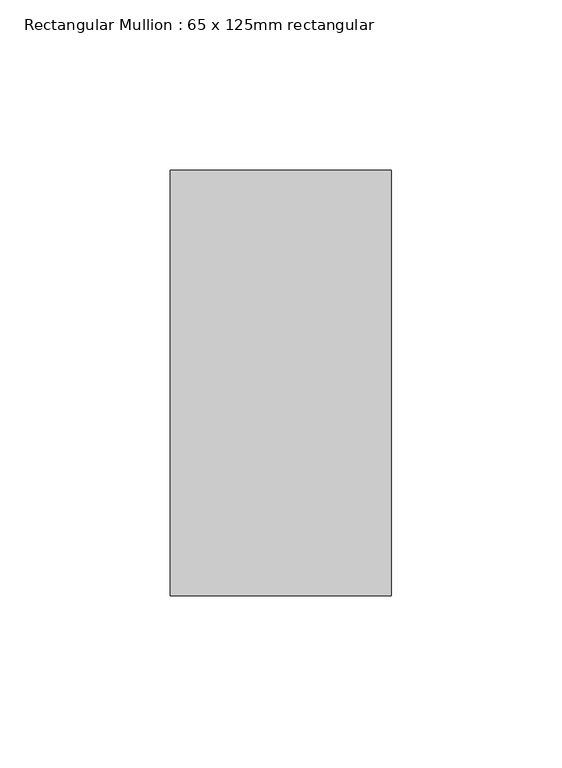
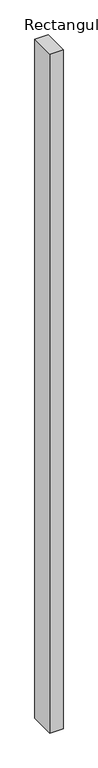
"""IFC4 building model written with IfcOpenShell, lengths in millimetres: member geometry, Rectangular Mullion : 65 x 125mm rectangular."""

from ifc_helpers import new_model, si_unit, frame, origin, place, context, project, spatial, polyline, outline, extrude, source, transform, mapped, element, save


def rectangular_mullion_65_x_125mm_rectangular_efb59fec(model_context):
    return source(origin(), model_context, "Body", "SweptSolid", [
        extrude(outline(polyline([(0.0, 62.5), (0.0, -62.5), (-65.0, -62.5), (-65.0, 62.5), (0.0, 62.5)])), frame((0.0, 0.0, -3500.0), z_axis=(0.0, 0.0, 1.0), x_axis=(1.0, 0.0, 0.0)), (0.0, 0.0, 1.0), 3500.0),
    ])


if __name__ == "__main__":
    model = new_model("IFC4")
    model_context = context("Model", 3, world=origin())
    ifc_project = project(units=[si_unit("LENGTHUNIT", "METRE", prefix="MILLI")], contexts=[model_context])
    site = spatial("IfcSite", under=ifc_project)
    building = spatial("IfcBuilding", under=site)
    placement = place(None, origin())
    rectangular_mullion_65_x_125mm_rectangular_shape = rectangular_mullion_65_x_125mm_rectangular_efb59fec(model_context)
    element("IfcMember", 1, ObjectType="Rectangular Mullion : 65 x 125mm rectangular", at=placement, inside=building, context=model_context, shape_type="MappedRepresentation", body=[
        mapped(rectangular_mullion_65_x_125mm_rectangular_shape, transform((0.0, 0.0, 0.0), x_axis=(1.0, 0.0, 0.0), y_axis=(0.0, 1.0, 0.0), z_axis=(0.0, 0.0, 1.0))),
    ])
    save(model, "model.ifc")

# Revit data of these elements
# Type "Rectangular Mullion : 65 x 125mm rectangular"
#   built-in parameter 1007304 = 0.410105 (stored number, unit not read)
#   built-in parameter 1007301 = 0.106627 (stored number, unit not read)
#   built-in parameter 1007300 = 0.106627 (stored number, unit not read)
# Element 1 (IfcMember, "Rectangular Mullion : 65 x 125mm rectangular")
#   Materials on its faces: "Aluminum"
# Materials
#   "Aluminum": class "Metal", colour RGB 244 245 246, transparency 0, Description = "Aluminum 6061", Cost = 0
